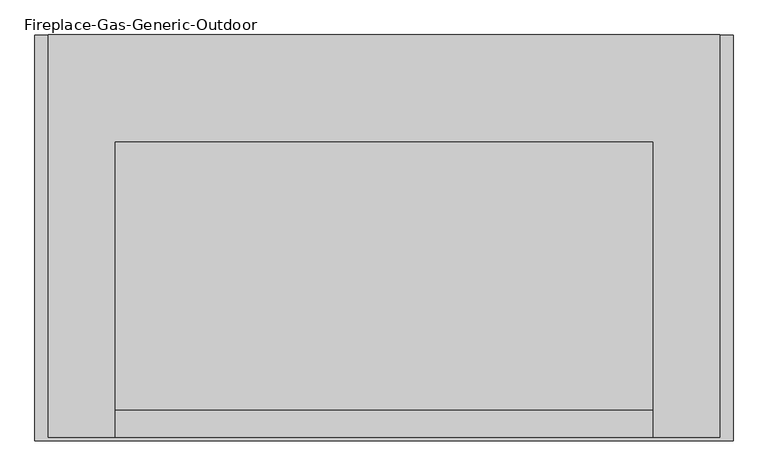
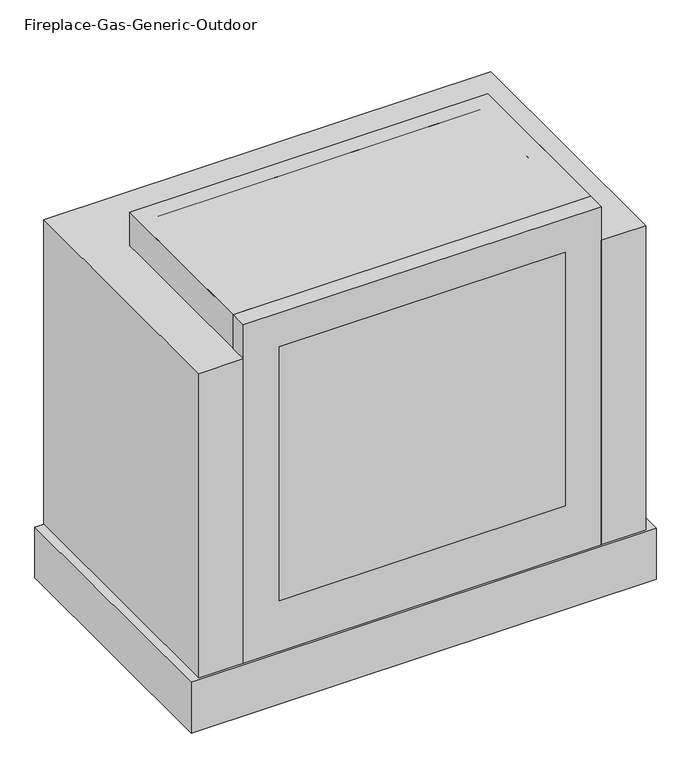
"""IFC4 building model written with IfcOpenShell, lengths in millimetres: proxy geometry, Fireplace-Gas-Generic-Outdoor : Liquid Propane."""

from ifc_helpers import new_model, si_unit, point, frame, origin, origin_with_axes, origin_2d, place, context, project, spatial, polyline, circle_curve, trimmed, segment, composite_curve, outline, extrude, source, transform, mapped, element, save


def fireplace_gas_generic_outdoor_4c8c5e7d(model_context):
    return source(origin(), model_context, "Body", "SweptSolid", [
        extrude(outline(composite_curve([segment(trimmed(circle_curve(origin_2d(), 76.2), [point((0.0, 76.2))], [point((1e-07, -76.2))], False, "CARTESIAN"), True, "CONTINUOUS"), segment(trimmed(circle_curve(origin_2d(), 76.2), [point((1e-07, -76.2))], [point((0.0, 76.2))], False, "CARTESIAN"), True, "CONTINUOUS")], self_intersect=False)), frame((-211.8574948, 123.6439192, 488.8127797), z_axis=(0.8364029855964028, -0.4636257455782089, 0.2923717047227273), x_axis=(-0.48480962024633606, -0.8746197071393964, 0.0)), (0.0, 0.0, 1.0), 457.2),
        extrude(outline(composite_curve([segment(trimmed(circle_curve(origin_2d(), 76.2), [point((0.0, 76.2))], [point((0.0, -76.2))], False, "CARTESIAN"), True, "CONTINUOUS"), segment(trimmed(circle_curve(origin_2d(), 76.2), [point((0.0, -76.2))], [point((0.0, 76.2))], False, "CARTESIAN"), True, "CONTINUOUS")], self_intersect=False)), frame((-219.1212604, 95.6001641, 377.6704224), z_axis=(0.9563047559630384, 0.0, 0.2923717047227272), x_axis=(0.0, -1.0, 0.0)), (0.0, 0.0, 1.0), 457.2),
        extrude(outline(composite_curve([segment(trimmed(circle_curve(origin_2d(), 76.2), [point((0.0, -76.2))], [point((0.0, 76.2))], False, "CARTESIAN"), True, "CONTINUOUS"), segment(trimmed(circle_curve(origin_2d(), 76.2), [point((0.0, 76.2))], [point((0.0, -76.2))], False, "CARTESIAN"), True, "CONTINUOUS")], self_intersect=False)), frame((218.8489393, -75.0720774, 379.7812831), z_axis=(-0.9848077530122076, 0.0, 0.17364817766693336), x_axis=(0.0, -1.0, 0.0)), (0.0, 0.0, 1.0), 457.2),
        extrude(outline(polyline([(406.4, -279.4), (-406.4, -279.4), (-406.4, -260.35), (406.4, -260.35), (406.4, -279.4)])), frame((0.0, 0.0, 304.8), z_axis=(0.0, 0.0, 1.0), x_axis=(1.0, 0.0, 0.0)), (0.0, 0.0, 1.0), 762.0),
        extrude(outline(polyline([(1168.4, 508.0), (1168.4, -508.0), (152.4, -508.0), (152.4, 508.0), (1168.4, 508.0)]), holes=[polyline([(1066.8, 406.4), (304.8, 406.4), (304.8, -406.4), (1066.8, -406.4), (1066.8, 406.4)])]), frame((0.0, -279.4, 0.0), z_axis=(0.0, 1.0, 0.0), x_axis=(0.0, 0.0, 1.0)), (0.0, 0.0, 1.0), 50.8),
        extrude(outline(polyline([(660.4, -285.75), (-660.4, -285.75), (-660.4, 482.6), (660.4, 482.6), (660.4, -285.75)])), origin_with_axes(), (0.0, 0.0, 1.0), 152.4),
        extrude(outline(polyline([(-508.0, -279.4), (-635.0, -279.4), (-635.0, 482.6), (635.0, 482.6), (635.0, -279.4), (508.0, -279.4), (508.0, 279.4), (-508.0, 279.4), (-508.0, -279.4)])), frame((0.0, 0.0, 152.4), z_axis=(0.0, 0.0, 1.0), x_axis=(1.0, 0.0, 0.0)), (0.0, 0.0, 1.0), 914.4),
        extrude(outline(polyline([(508.0, -279.4), (-508.0, -279.4), (-508.0, 279.4), (508.0, 279.4), (508.0, -279.4)])), frame((0.0, 0.0, 1066.8), z_axis=(0.0, 0.0, 1.0), x_axis=(1.0, 0.0, 0.0)), (0.0, 0.0, 1.0), 101.6),
        extrude(outline(polyline([(-457.2, 228.6), (457.2, 228.6), (457.2, -228.6), (-457.2, -228.6), (-457.2, 228.6)])), frame((0.0, 0.0, 152.4), z_axis=(0.0, 0.0, 1.0), x_axis=(1.0, 0.0, 0.0)), (0.0, 0.0, 1.0), 152.4),
        extrude(outline(polyline([(-457.2, 228.6), (-457.2, -228.6), (-508.0, -228.6), (-508.0, 279.4), (508.0, 279.4), (508.0, -228.6), (457.2, -228.6), (457.2, 228.6), (-457.2, 228.6)])), frame((0.0, 0.0, 152.4), z_axis=(0.0, 0.0, 1.0), x_axis=(1.0, 0.0, 0.0)), (0.0, 0.0, 1.0), 1016.0),
    ])


if __name__ == "__main__":
    model = new_model("IFC4")
    model_context = context("Model", 3, world=origin())
    ifc_project = project(units=[si_unit("LENGTHUNIT", "METRE", prefix="MILLI")], contexts=[model_context])
    site = spatial("IfcSite", under=ifc_project)
    building = spatial("IfcBuilding", under=site)
    placement = place(None, origin())
    fireplace_gas_generic_outdoor_shape = fireplace_gas_generic_outdoor_4c8c5e7d(model_context)
    element("IfcBuildingElementProxy", 1, Name="Fireplace-Gas-Generic-Outdoor : Liquid Propane", ObjectType="Fireplace-Gas-Generic-Outdoor : Liquid Propane", at=placement, inside=building, context=model_context, shape_type="MappedRepresentation", body=[
        mapped(fireplace_gas_generic_outdoor_shape, transform((0.0, 0.0, 0.0), x_axis=(1.0, 0.0, 0.0), y_axis=(0.0, 1.0, 0.0), z_axis=(0.0, 0.0, 1.0))),
    ])
    save(model, "model.ifc")

# Revit data of these elements
# Type "Fireplace-Gas-Generic-Outdoor : Liquid Propane"
#   Type Mark = "Majastic Vented Fireplace"
#   COBie.Type.CreatedBy = "design@eagle.com"
#   COBie.Type.CreatedOn = "2016-10-27T05:31:12"
#   COBie.Type.Name = "Fireplace-Gas-Generic-Outdoor_Liquid Propane_Majastic Vented Fireplace"
#   COBie.Type.Category = "n/a"
#   COBie.Type.Description = "Fireplace-Gas-Generic-Outdoor_Liquid Propane"
#   COBie.Type.Manufacturer = "Generic"
#   COBie.Type.ModelNumber = "Gas Outdoor Fireplace"
#   Type Comments = "Optional Liquid Propane or Natural Gas"
#   Model = "Gas Outdoor Fireplace"
#   Manufacturer = "Generic"
#   Gas Connector Description = ""
#   Electrical Connector Description = ""
#   OmniClass Title = "Fireplaces"
#   OmniClass Number = "23.40.20.34.14"
#   Description = "Gas Fireplace with Electrical Ignition"
#   Connector Description Electrical = "Power Supply"
#   COBie.Type.ReplacementCost = 0
#   Width of Insert = 3' - 4"
#   Width = 3' - 6"
#   Voltage [instance default] = 0 V
#   Power Factor [instance default] = 1
#   Height = 3' - 0"
#   Gas Pressure Drop = 0.00 psi
#   Gas Connection Radius = 1/2"
#   Depth = 2' - 6"
#   CTRL Width = 4' - 2"
#   CTRL Height of Base = 0' - 6"
#   CTRL Depth = 2' - 6"
#   Overall Width = 4' - 4"
#   Overall Height = 4' - 1"
#   Overall Depth = 2' - 6 1/4"
#   Height of Insert = 3' - 4"
#   Glass Width = 2' - 8"
#   Glass Height = 2' - 6"
#   Depth of Insert = 1' - 10"
#   Base Offset Width = 1"
#   Base Height = 6"
#   Apparent Load = 0 VA
#   Actual Heater Gas Flow = 0 GPM
#   COBie.Type = yes
#   Natural Gas [instance default] = no
#   Liquid Propane [instance default] = yes
#   Number of Poles [instance default] = 1
#   Top Counter Material [instance default] = Stone - Generic - Marble - White Coarse Polished
#   Log Materia [instance default] = Wood - Generic - Log
#   Frame Material [instance default] = Iron - Generic - Black
#   Mantel Material [instance default] = Stone - Generic - Stacked
#   Glazing Material [instance default] = Glass - Generic - Gray
#   Body Material [instance default] = Stone - Generic - Stacked
#   Emit Shape Visible in Rendering = no
# Element 1 (IfcBuildingElementProxy, "Fireplace-Gas-Generic-Outdoor : Liquid Propane")
#   Materials on its faces: "Stone - Generic - Stacked", "Wood - Generic - Log", "Iron - Generic - Black", "Glass - Generic - Gray"
# Materials
#   "Stone - Generic - Marble - White Coarse Polished": class "Stone", colour RGB 171 182 182, transparency 0
#   "Wood - Generic - Log": class "Wood", colour RGB 137 123 92, transparency 0
#   "Iron - Generic - Black": class "Metal", colour RGB 10 10 10, transparency 0
#   "Stone - Generic - Stacked": class "Stone", colour RGB 145 127 91, transparency 0
#   "Glass - Generic - Gray": class "Glass", colour RGB 115 114 120, transparency 0.95
